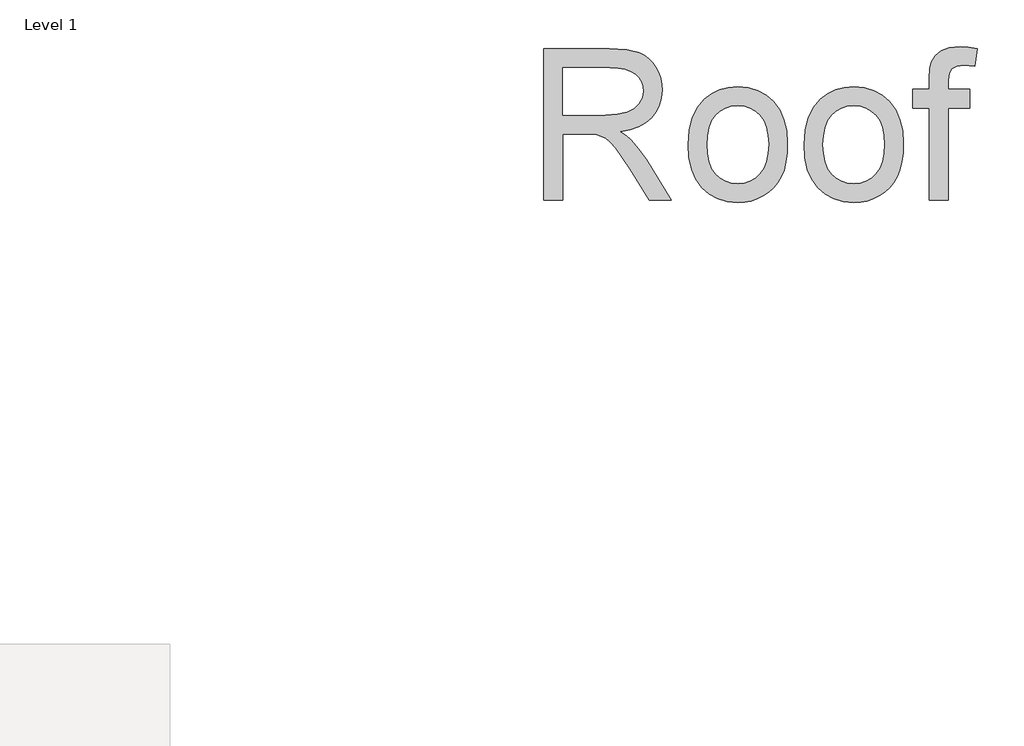
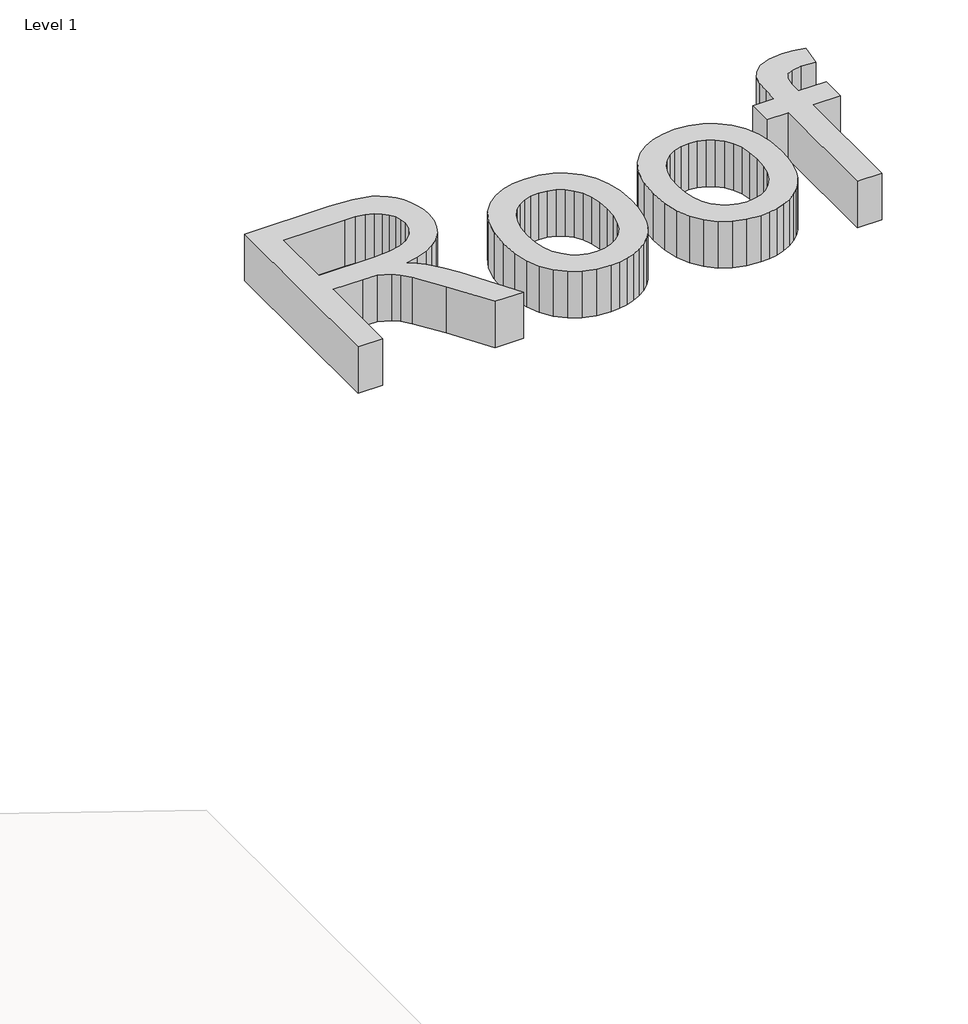
# One storey, part 8 of 42: 1 proxy.
"""IFC4 building model written with IfcOpenShell, lengths in millimetres."""

from ifc_helpers import new_model, si_unit, origin, origin_with_axes, place, context, project, spatial, polyline, outline, extrude, element, save

model = new_model("IFC4")

# Units and contexts
model_context = context("Model", 3, world=origin())
ifc_project = project(units=[si_unit("LENGTHUNIT", "METRE", prefix="MILLI")], contexts=[model_context])

# Site, building, storey
site = spatial("IfcSite", under=ifc_project)
building = spatial("IfcBuilding", under=site)
storey = spatial("IfcBuildingStorey", under=building, Name="Level 1", Elevation=0.0)

# Proxy
placement = place(None, origin())
element("IfcBuildingElementProxy", 1, Name="24\" Arial", ObjectType="24\" Arial", at=placement, inside=storey, context=model_context, shape_type="SweptSolid", body=[
    extrude(outline(polyline([(-9142.0272497, -3275.1761465), (-9142.0272497, -2666.0419584), (-8879.5463312, -2666.0419584), (-8808.9999371, -2670.1501937), (-8757.6748793, -2682.4748997), (-8737.86798, -2692.2714609), (-8720.1616715, -2705.2282031), (-8704.5559541, -2721.3451264), (-8691.0508275, -2740.6222307), (-8680.1528502, -2762.0231625), (-8672.3685808, -2784.5115684), (-8667.6980191, -2808.0874483), (-8666.1411652, -2832.7508023), (-8668.7204306, -2864.0365945), (-8676.4582268, -2892.7570633), (-8689.3545538, -2918.9122086), (-8707.4094116, -2942.5020306), (-8730.8551665, -2962.7736624), (-8759.9241846, -2978.9742375), (-8794.6164661, -2991.1037559), (-8834.9320108, -2999.1622175), (-8809.8364556, -3015.5579803), (-8791.65612, -3031.7306714), (-8760.4632743, -3068.7233788), (-8729.9396434, -3110.1031609), (-8628.3677073, -3275.1761465), (-8716.8527761, -3275.1761465), (-8796.1175521, -3148.9176197), (-8853.3725966, -3065.3401261), (-8874.6573453, -3040.9695536), (-8893.5998422, -3025.8564525), (-8929.8117989, -3011.3567984), (-8973.9799761, -3008.6799392), (-9065.8854762, -3008.6799392), (-9065.8854762, -3275.1761465), (-9142.0272497, -3275.1761465)]), holes=[polyline([(-9065.8854762, -2932.5381657), (-8895.4587722, -2932.5381657), (-8846.5131448, -2929.8427171), (-8808.5352046, -2921.7563716), (-8779.9448609, -2907.7400392), (-8759.1620233, -2887.2546304), (-8746.5027099, -2862.4750933), (-8742.2829388, -2835.576376), (-8744.2952305, -2816.104084), (-8750.3321057, -2798.4349542), (-8760.3935645, -2782.5689865), (-8774.4796067, -2768.5061809), (-8792.9155451, -2756.9901095), (-8816.0266926, -2748.7643441), (-8843.813049, -2743.8288849), (-8876.2746144, -2742.1837319), (-9065.8854762, -2742.1837319), (-9065.8854762, -2932.5381657)])]), origin_with_axes(), (0.0, 0.0, 1.0), 152.4),
    extrude(outline(polyline([(-8561.4462267, -3051.5096868), (-8557.3286967, -2993.5761328), (-8544.9761067, -2943.6545672), (-8524.3884568, -2901.7449899), (-8495.5657468, -2867.8474011), (-8466.5478493, -2846.1815717), (-8434.5184851, -2830.7059793), (-8399.4776542, -2821.4206239), (-8361.4253568, -2818.3255054), (-8319.4181857, -2822.094486), (-8281.4355981, -2833.4014278), (-8247.477594, -2852.2463309), (-8217.5441734, -2878.6291952), (-8193.1131857, -2911.6577342), (-8175.6624801, -2950.4396617), (-8165.1920568, -2994.9749776), (-8161.7019157, -3045.2636819), (-8163.2448276, -3086.0207226), (-8167.8735633, -3122.1862061), (-8175.5881229, -3153.7601324), (-8186.3885063, -3180.7425016), (-8200.1399411, -3204.0488367), (-8216.7076549, -3224.5946607), (-8236.0916477, -3242.3799737), (-8258.2919194, -3257.4047755), (-8282.4440677, -3269.3437536), (-8307.68369, -3277.871595), (-8334.0107863, -3282.9882999), (-8361.4253568, -3284.6938682), (-8404.0459747, -3280.9388296), (-8442.381759, -3269.6737136), (-8476.4327096, -3250.8985205), (-8506.1988265, -3224.61325), (-8530.3695641, -3191.2640455), (-8547.6343766, -3151.2970501), (-8557.9932641, -3104.7122639), (-8561.4462267, -3051.5096868)]), holes=[polyline([(-8485.3044531, -3051.3609724), (-8483.1016211, -3088.2932645), (-8476.4931249, -3120.2715081), (-8465.4789645, -3147.2957033), (-8450.05914, -3169.3658499), (-8431.3025361, -3186.509832), (-8410.2780376, -3198.7555335), (-8386.9856445, -3206.1029544), (-8361.4253568, -3208.5520947), (-8335.9951941, -3206.0890124), (-8312.7957475, -3198.6997656), (-8291.8270169, -3186.3843542), (-8273.0890023, -3169.1427783), (-8257.6691778, -3146.8542074), (-8246.6550175, -3119.397811), (-8240.0465213, -3086.7735892), (-8237.8436892, -3048.981542), (-8240.0604633, -3013.2203758), (-8246.7107854, -2982.0786506), (-8257.7946556, -2955.5563666), (-8273.3120739, -2933.6535237), (-8292.1197984, -2916.5095416), (-8313.074587, -2904.2638401), (-8336.1764398, -2896.9164192), (-8361.4253568, -2894.4672789), (-8386.9856445, -2896.9071246), (-8410.2780376, -2904.2266615), (-8431.3025361, -2916.4258897), (-8450.05914, -2933.5048093), (-8465.4789645, -2955.5098934), (-8476.4931249, -2982.4876152), (-8483.1016211, -3014.4379749), (-8485.3044531, -3051.3609724)])]), origin_with_axes(), (0.0, 0.0, 1.0), 152.4),
    extrude(outline(polyline([(-8095.0778639, -3051.5096868), (-8090.9603339, -2993.5761328), (-8078.6077439, -2943.6545672), (-8058.020094, -2901.7449899), (-8029.197384, -2867.8474011), (-8000.1794865, -2846.1815717), (-7968.1501223, -2830.7059793), (-7933.1092914, -2821.4206239), (-7895.056994, -2818.3255054), (-7853.0498229, -2822.094486), (-7815.0672353, -2833.4014278), (-7781.1092312, -2852.2463309), (-7751.1758106, -2878.6291952), (-7726.7448229, -2911.6577342), (-7709.2941173, -2950.4396617), (-7698.823694, -2994.9749776), (-7695.3335529, -3045.2636819), (-7696.8764648, -3086.0207226), (-7701.5052006, -3122.1862061), (-7709.2197601, -3153.7601324), (-7720.0201435, -3180.7425016), (-7733.7715783, -3204.0488367), (-7750.3392921, -3224.5946607), (-7769.7232849, -3242.3799737), (-7791.9235566, -3257.4047755), (-7816.0757049, -3269.3437536), (-7841.3153272, -3277.871595), (-7867.6424235, -3282.9882999), (-7895.056994, -3284.6938682), (-7937.677612, -3280.9388296), (-7976.0133962, -3269.6737136), (-8010.0643468, -3250.8985205), (-8039.8304637, -3224.61325), (-8064.0012013, -3191.2640455), (-8081.2660138, -3151.2970501), (-8091.6249014, -3104.7122639), (-8095.0778639, -3051.5096868)]), holes=[polyline([(-8018.9360903, -3051.3609724), (-8016.7332583, -3088.2932645), (-8010.1247621, -3120.2715081), (-7999.1106017, -3147.2957033), (-7983.6907772, -3169.3658499), (-7964.9341733, -3186.509832), (-7943.9096748, -3198.7555335), (-7920.6172817, -3206.1029544), (-7895.056994, -3208.5520947), (-7869.6268313, -3206.0890124), (-7846.4273847, -3198.6997656), (-7825.4586541, -3186.3843542), (-7806.7206395, -3169.1427783), (-7791.3008151, -3146.8542074), (-7780.2866547, -3119.397811), (-7773.6781585, -3086.7735892), (-7771.4753264, -3048.981542), (-7773.6921005, -3013.2203758), (-7780.3424226, -2982.0786506), (-7791.4262928, -2955.5563666), (-7806.9437111, -2933.6535237), (-7825.7514356, -2916.5095416), (-7846.7062242, -2904.2638401), (-7869.808077, -2896.9164192), (-7895.056994, -2894.4672789), (-7920.6172817, -2896.9071246), (-7943.9096748, -2904.2266615), (-7964.9341733, -2916.4258897), (-7983.6907772, -2933.5048093), (-7999.1106017, -2955.5098934), (-8010.1247621, -2982.4876152), (-8016.7332583, -3014.4379749), (-8018.9360903, -3051.3609724)])]), origin_with_axes(), (0.0, 0.0, 1.0), 152.4),
    extrude(outline(polyline([(-7590.6386143, -3275.1761465), (-7590.6386143, -2903.9850006), (-7657.2626661, -2903.9850006), (-7657.2626661, -2827.8432271), (-7590.6386143, -2827.8432271), (-7590.6386143, -2782.7827635), (-7588.6309699, -2745.4926273), (-7582.6080366, -2719.2817141), (-7567.2904533, -2693.9630872), (-7543.6448635, -2673.9238216), (-7510.5559092, -2660.8741329), (-7466.9082323, -2656.5242367), (-7433.8564566, -2658.6062383), (-7397.4586069, -2664.8522431), (-7408.612187, -2736.2351558), (-7452.4829354, -2732.6660102), (-7481.4264758, -2735.8261912), (-7500.4433299, -2745.3067343), (-7510.9834631, -2763.4127127), (-7514.4968408, -2792.4491995), (-7514.4968408, -2827.8432271), (-7428.8373456, -2827.8432271), (-7428.8373456, -2903.9850006), (-7514.4968408, -2903.9850006), (-7514.4968408, -3275.1761465), (-7590.6386143, -3275.1761465)])), origin_with_axes(), (0.0, 0.0, 1.0), 152.4),
])

save(model, "model.ifc")

# Revit data of these elements
# Element 1 (IfcBuildingElementProxy, "24\" Arial")
#   Phase Created = New Construction
